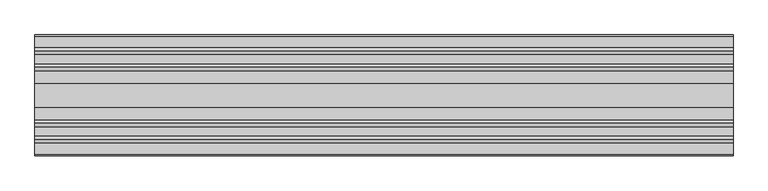
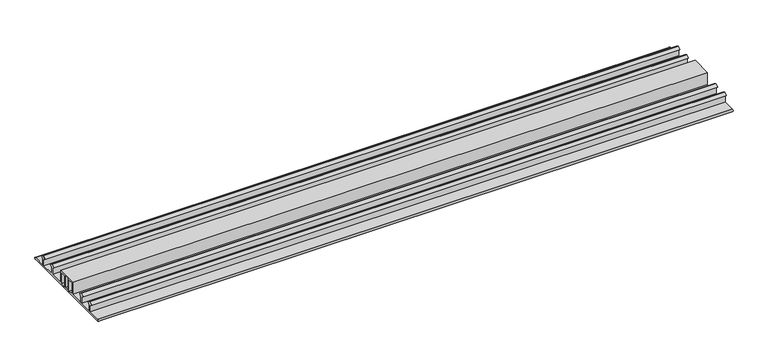
"""IFC4 building model written with IfcOpenShell, lengths in millimetres: proxy geometry, TN_ПВХ_ТПО_Гидрошпонка ТехноНИКОЛЬ : ПВХ Гидрошпонка ТехноНИКОЛЬ EM-260/50."""

from ifc_helpers import new_model, si_unit, point, frame, frame_2d, origin, place, context, project, spatial, polyline, circle_curve, trimmed, segment, composite_curve, outline, extrude, source, transform, mapped, element, save


def specialty_equipment_5da421ea(model_context):
    return source(origin(), model_context, "Body", "SweptSolid", [
        extrude(outline(composite_curve([segment(polyline([(127.5, 0.0), (-127.5, 0.0)]), True, "CONTINUOUS"), segment(trimmed(circle_curve(frame_2d((-127.5, 2.5)), 2.5), [point((-127.5, 0.0))], [point((-127.5, 5.0))], False, "CARTESIAN"), True, "CONTINUOUS"), segment(polyline([(-127.5, 5.0), (-97.0456593, 5.0), (-97.0456593, 20.0), (-101.8901067, 23.875134), (-95.0, 28.0), (-88.1098933, 23.875134), (-92.9543407, 20.0), (-92.9543407, 5.0), (-62.0456593, 5.0), (-62.0456593, 20.0), (-66.8901067, 23.875134), (-60.0, 28.0), (-53.1098933, 23.875134), (-57.9543407, 20.0), (-57.9543407, 5.0), (-25.0, 5.0), (-25.0, 35.0), (25.0, 35.0), (25.0, 5.0), (57.9543407, 5.0), (57.9543407, 20.0), (53.1098933, 23.875134), (60.0, 28.0), (66.8901067, 23.875134), (62.0456593, 20.0), (62.0456593, 5.0), (92.9543407, 5.0), (92.9543407, 20.0), (88.1098933, 23.875134), (95.0, 28.0), (101.8901067, 23.875134), (97.0456593, 20.0), (97.0456593, 5.0), (127.5, 5.0)]), True, "CONTINUOUS"), segment(trimmed(circle_curve(frame_2d((127.5, 2.5)), 2.5), [point((127.5, 5.0))], [point((127.5, 0.0))], False, "CARTESIAN"), True, "CONTINUOUS")], self_intersect=False), holes=[polyline([(-20.0, 30.0), (-20.0, 5.0), (-9.2211828, 2.9048102), (-9.2211828, 30.0), (-20.0, 30.0)]), polyline([(20.0, 5.0), (20.0, 30.0), (9.2211828, 30.0), (9.2211828, 2.9048102), (20.0, 5.0)]), polyline([(-4.2211828, 5.0), (4.2211828, 5.0), (4.2211828, 34.0), (-4.2211828, 34.0), (-4.2211828, 5.0)])]), frame((0.0, 0.0, 0.0), z_axis=(1.0, 0.0, 0.0), x_axis=(0.0, 1.0, 0.0)), (0.0, 0.0, 1.0), 1500.0),
    ])


if __name__ == "__main__":
    model = new_model("IFC4")
    model_context = context("Model", 3, world=origin())
    ifc_project = project(units=[si_unit("LENGTHUNIT", "METRE", prefix="MILLI")], contexts=[model_context])
    site = spatial("IfcSite", under=ifc_project)
    building = spatial("IfcBuilding", under=site)
    placement = place(None, origin())
    specialty_equipment_shape = specialty_equipment_5da421ea(model_context)
    element("IfcBuildingElementProxy", 1, Name="TN_ПВХ_ТПО_Гидрошпонка ТехноНИКОЛЬ : ПВХ Гидрошпонка ТехноНИКОЛЬ EM-260/50", ObjectType="TN_ПВХ_ТПО_Гидрошпонка ТехноНИКОЛЬ : ПВХ Гидрошпонка ТехноНИКОЛЬ EM-260/50", at=placement, inside=building, context=model_context, shape_type="MappedRepresentation", body=[
        mapped(specialty_equipment_shape, transform((0.0, 0.0, 0.0), x_axis=(1.0, 0.0, 0.0), y_axis=(0.0, 1.0, 0.0), z_axis=(0.0, 0.0, 1.0))),
    ])
    save(model, "model.ifc")

# Revit data of these elements
# Type "TN_ПВХ_ТПО_Гидрошпонка ТехноНИКОЛЬ : ПВХ Гидрошпонка ТехноНИКОЛЬ EM-260/50"
#   Description = "Опалубочная деформационная ПВХ гидрошпонка. Ширина деформационного узла 50 мм.  Применяется для герметизации деформационных швов при строительстве заглубленных и подземных сооружений"
#   Type Comments = "п.м."
#   Manufacturer = "ТехноНИКОЛЬ"
#   URL = "https://shop.tn.ru/pvh-gidroshponka-em-260-50-10-m-rul"
#   ADSK_Примечание = ""
#   ADSK_Обозначение [instance default] = "ТехноНИКОЛЬ"
#   ADSK_Наименование = "ПВХ Гидрошпонка ТехноНИКОЛЬ EM-260/50"
#   ADSK_Масса_Текст = ""
#   ADSK_Марка = ""
#   ADSK_Код изделия = "499186"
#   ADSK_Завод-изготовитель [instance default] = "ТехноНИКОЛЬ"
#   ADSK_Единица измерения [instance default] = "п.м."
#   ADSK_Группирование = "Гидрошпонки"
#   ADSK_URL страницы изделия = "https://shop.tn.ru/pvh-gidroshponka-em-260-50-10-m-rul"
#   ADSK_URL документации изделия = "https://nav.tn.ru/upload/iblock/67f/Katalog-i-rekomendatsii-po-primeneniyu_Gidroshponki-TEKHNONIKOL.PDF"
#   built-in parameter 1001306 [instance default] = 3.28084 (stored number, unit not read)
#   ADSK_Размер_Длина [instance default] = 1000 mm
#   ADSK_Количество [instance default] = 1
#   ПВХ_ТПО Гидрошпонка ТехноНИКОЛЬ EC-320-4 = no
#   ПВХ Гидрошпонка ТехноНИКОЛЬ IM-260/50 = no
#   ПВХ Гидрошпонка ТехноНИКОЛЬ IM-240/20 = no
#   ПВХ Гидрошпонка ТехноНИКОЛЬ IC-240-6 = no
#   ПВХ Гидрошпонка ТехноНИКОЛЬ IC-125-2SP = no
#   ПВХ Гидрошпонка ТехноНИКОЛЬ EM-260/50 = yes
#   ПВХ Гидрошпонка ТехноНИКОЛЬ EM-260/20 = no
#   ПВХ Гидрошпонка ТехноНИКОЛЬ EC-320-4 = no
#   ПВХ Гидрошпонка ТехноНИКОЛЬ EC-220-3 = no
#   ПВХ_ТПО Гидрошпонка ТехноНИКОЛЬ EC-220-3 = no
#   ПВХ Гидрошпонка ТехноНИКОЛЬ IC-240-2 = no
#   Материал = TN_ПВХ_Черный
#   Default Elevation = 0
# Element 1 (IfcBuildingElementProxy, "TN_ПВХ_ТПО_Гидрошпонка ТехноНИКОЛЬ : ПВХ Гидрошпонка ТехноНИКОЛЬ EM-260/50")
#   built-in parameter 1001306 = 4.92126 (stored number, unit not read)
#   ADSK_Размер_Длина = 1500 mm
#   ADSK_Количество = 1.5
#   Materials on its faces: "TN_ПВХ_Черный"
# Materials
#   "TN_ПВХ_Черный": class "Типовые", colour RGB 48 48 48, transparency 0, Cost = 0
